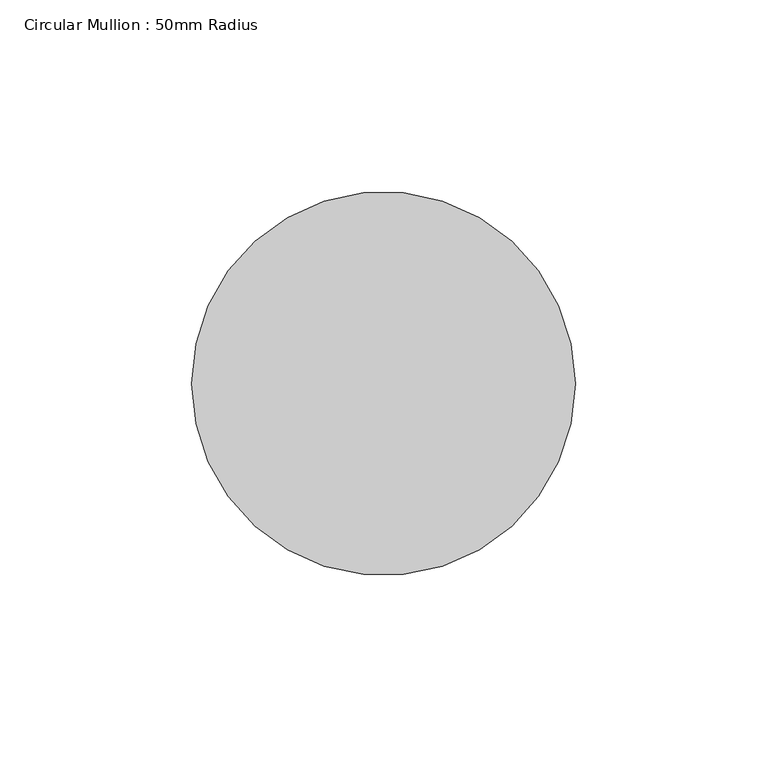
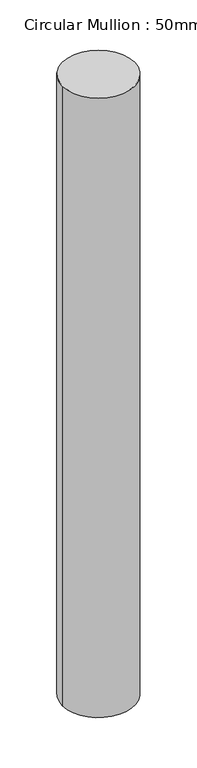
"""IFC4 building model written with IfcOpenShell, lengths in millimetres: member geometry, Circular Mullion : 50mm Radius."""

from ifc_helpers import new_model, si_unit, point, frame, origin, origin_2d, place, context, project, spatial, circle_curve, trimmed, segment, composite_curve, outline, extrude, source, transform, mapped, element, save


def circular_mullion_50mm_radius_f3fed7ef(model_context):
    return source(origin(), model_context, "Body", "SweptSolid", [
        extrude(outline(composite_curve([segment(trimmed(circle_curve(origin_2d(), 50.0), [point((50.0, 0.0))], [point((-50.0, 0.0))], False, "CARTESIAN"), True, "CONTINUOUS"), segment(trimmed(circle_curve(origin_2d(), 50.0), [point((-50.0, 0.0))], [point((50.0, 0.0))], False, "CARTESIAN"), True, "CONTINUOUS")], self_intersect=False)), frame((0.0, 0.0, -908.7402344), z_axis=(0.0, 0.0, 1.0), x_axis=(1.0, 0.0, 0.0)), (0.0, 0.0, 1.0), 908.7402344),
    ])


if __name__ == "__main__":
    model = new_model("IFC4")
    model_context = context("Model", 3, world=origin())
    ifc_project = project(units=[si_unit("LENGTHUNIT", "METRE", prefix="MILLI")], contexts=[model_context])
    site = spatial("IfcSite", under=ifc_project)
    building = spatial("IfcBuilding", under=site)
    placement = place(None, origin())
    circular_mullion_50mm_radius_shape = circular_mullion_50mm_radius_f3fed7ef(model_context)
    element("IfcMember", 1, ObjectType="Circular Mullion : 50mm Radius", at=placement, inside=building, context=model_context, shape_type="MappedRepresentation", body=[
        mapped(circular_mullion_50mm_radius_shape, transform((0.0, 0.0, 0.0), x_axis=(1.0, 0.0, 0.0), y_axis=(0.0, 1.0, 0.0), z_axis=(0.0, 0.0, 1.0))),
    ])
    save(model, "model.ifc")

# Revit data of these elements
# Type "Circular Mullion : 50mm Radius"
#   built-in parameter 1007350 = 0.164042 (stored number, unit not read)
# Element 1 (IfcMember, "Circular Mullion : 50mm Radius")
#   Materials on its faces: "Aluminium"
# Materials
#   "Aluminium": class "Metal", colour RGB 247 247 247, transparency 0, Description = "Aluminium 6061", Cost = 0
